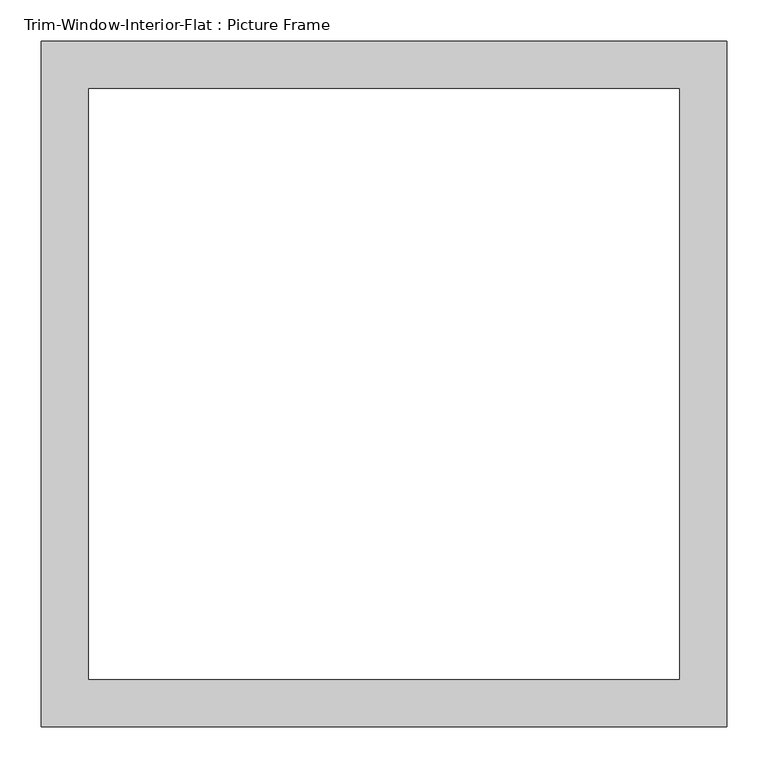
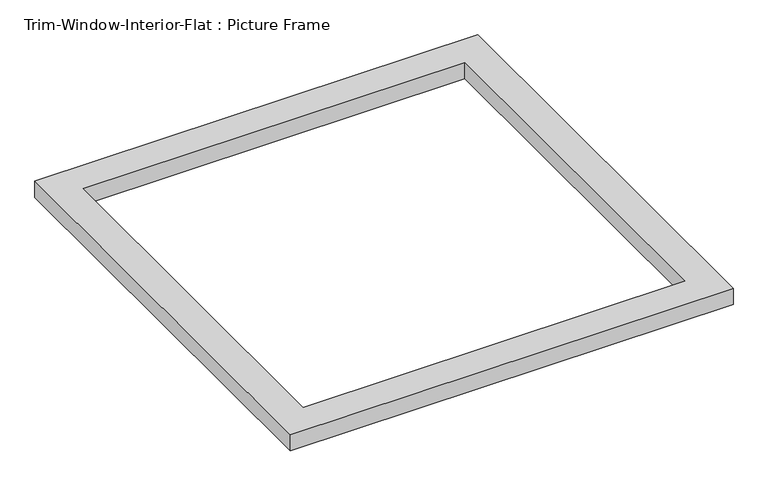
"""IFC4 building model written with IfcOpenShell, lengths in millimetres: proxy geometry, Trim-Window-Interior-Flat : Picture Frame."""

from ifc_helpers import new_model, si_unit, origin, origin_with_axes, place, context, project, spatial, polyline, outline, extrude, source, transform, mapped, element, save


def trim_window_interior_flat_picture_frame_9d512eb7(model_context):
    return source(origin(), model_context, "Body", "SweptSolid", [
        extrude(outline(polyline([(412.75, 44.45), (412.75, -781.05), (-412.75, -781.05), (-412.75, 44.45), (412.75, 44.45)]), holes=[polyline([(355.6, -12.7), (-355.6, -12.7), (-355.6, -723.9), (355.6, -723.9), (355.6, -12.7)])]), origin_with_axes(), (0.0, 0.0, 1.0), 31.75),
    ])


if __name__ == "__main__":
    model = new_model("IFC4")
    model_context = context("Model", 3, world=origin())
    ifc_project = project(units=[si_unit("LENGTHUNIT", "METRE", prefix="MILLI")], contexts=[model_context])
    site = spatial("IfcSite", under=ifc_project)
    building = spatial("IfcBuilding", under=site)
    placement = place(None, origin())
    trim_window_interior_flat_picture_frame_shape = trim_window_interior_flat_picture_frame_9d512eb7(model_context)
    element("IfcBuildingElementProxy", 1, Name="Trim-Window-Interior-Flat : Picture Frame", ObjectType="Trim-Window-Interior-Flat : Picture Frame", at=placement, inside=building, context=model_context, shape_type="MappedRepresentation", body=[
        mapped(trim_window_interior_flat_picture_frame_shape, transform((0.0, 0.0, 0.0), x_axis=(1.0, 0.0, 0.0), y_axis=(0.0, 1.0, 0.0), z_axis=(0.0, 0.0, 1.0))),
    ])
    save(model, "model.ifc")

# Revit data of these elements
# Type "Trim-Window-Interior-Flat : Picture Frame"
#   Trim Thickness_Picture Frame = 0' - 1 1/4"
#   Trim Width = 0' - 2 1/4"
#   Trim Thickness_with Sill = 0' - 0 3/4"
#   Sill Thickness = 0' - 1 1/4"
#   Opening Width [instance default] = 2' - 0"
#   Opening Height [instance default] = 3' - 0"
#   Default Elevation = 4' - 0"
#   Sill = no
#   Picture Frame = yes
#   Trim Material [instance default] = none
# Element 1 (IfcBuildingElementProxy, "Trim-Window-Interior-Flat : Picture Frame")
#   Opening Width = 2' - 5"
#   Opening Height = 2' - 5"
#   Trim Material = Wood - Stained
#   Materials on its faces: "Wood - Stained"
# Materials
#   "Wood - Stained": class "Wood", colour RGB 224 178 126, transparency 0, Cost = 0
